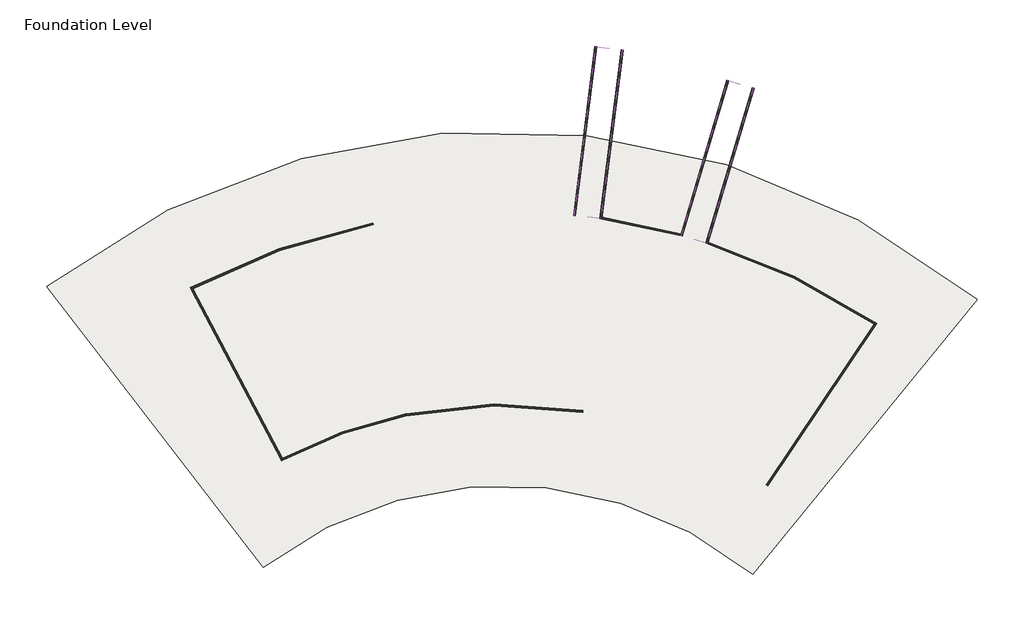
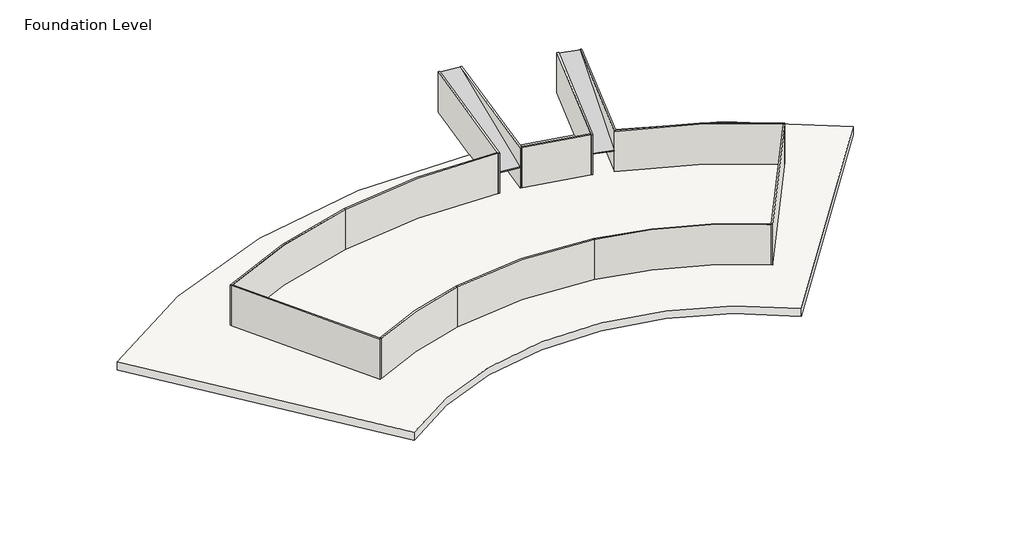
# One storey: 14 walls, 2 ramps, 1 slab.
"""IFC4 building model written with IfcOpenShell, lengths in millimetres."""

import ifcopenshell
import ifcopenshell.guid

model = None  # the IFC model being written
_history = None  # IfcOwnerHistory: only IFC2X3 demands one
_inside = {}  # id of a spatial element -> (the spatial element, [elements in it])
_under = {}  # id of a project, library or spatial element -> (it, [spatial elements below it])
_declared = {}  # id of a project -> (the project, [libraries it declares])
_typed = {}  # id of a type object -> (the type object, [elements of that type])
_made_of = {}  # id of a material, layer set ... -> (it, [elements and type objects made of it])


def new_model(schema):
    """Start an empty IFC model of exactly this schema.

    Asked for "IFC4X3", IfcOpenShell would pick the latest addendum, in which some entities
    have other attributes; the version numbers below select the first issue.
    IFC2X3 requires an IfcOwnerHistory on every rooted entity: one is made here for all.
    """
    global model, _history
    if schema == "IFC4X3":
        model = ifcopenshell.file(schema_version=(4, 3, 0, 0))
    else:
        model = ifcopenshell.file(schema=schema)
    _inside.clear()
    _under.clear()
    _declared.clear()
    _typed.clear()
    _made_of.clear()
    _history = None
    if model.schema == "IFC2X3":
        org = make("IfcOrganization", Name="unknown")
        user = make(
            "IfcPersonAndOrganization",
            ThePerson=make("IfcPerson", FamilyName="unknown"),
            TheOrganization=org,
        )
        app = make(
            "IfcApplication",
            ApplicationDeveloper=org,
            Version="unknown",
            ApplicationFullName="unknown",
            ApplicationIdentifier="unknown",
        )
        _history = make(
            "IfcOwnerHistory",
            OwningUser=user,
            OwningApplication=app,
            ChangeAction="ADDED",
            CreationDate=0,
        )
    return model


def make(cls, **values):
    """One entity of the class cls with the attributes given. An attribute that is None is left unset."""
    return model.create_entity(
        cls, **{name: value for name, value in values.items() if value is not None}
    )


def rooted(cls, **values):
    """An entity with a GlobalId (a new one), such as an element, a storey or a relation."""
    return make(cls, GlobalId=ifcopenshell.guid.new(), OwnerHistory=_history, **values)


def si_unit(unit_type, name, prefix=None):
    """IfcSIUnit, for example si_unit("LENGTHUNIT", "METRE", prefix="MILLI")."""
    return make("IfcSIUnit", UnitType=unit_type, Prefix=prefix, Name=name)


def assignment(units):
    """IfcUnitAssignment: the units of a project."""
    return None if units is None else make("IfcUnitAssignment", Units=units)


def point(xyz):
    """IfcCartesianPoint."""
    return None if xyz is None else make("IfcCartesianPoint", Coordinates=xyz)


def direction(xyz):
    """IfcDirection."""
    return None if xyz is None else make("IfcDirection", DirectionRatios=xyz)


def frame(location, z_axis=None, x_axis=None):
    """IfcAxis2Placement3D, a coordinate frame: its origin and axes. An axis left out is left unset."""
    return make(
        "IfcAxis2Placement3D",
        Location=point(location),
        Axis=direction(z_axis),
        RefDirection=direction(x_axis),
    )


def frame_2d(location, x_axis=None):
    """IfcAxis2Placement2D, a coordinate frame in the plane: its origin and x axis."""
    return make(
        "IfcAxis2Placement2D", Location=point(location), RefDirection=direction(x_axis)
    )


def origin():
    """The frame at (0, 0, 0) with its axes left unset."""
    return frame((0.0, 0.0, 0.0))


def origin_2d():
    """The frame at (0, 0) in the plane with its x axis left unset."""
    return frame_2d((0.0, 0.0))


def place(relative_to, where):
    """IfcLocalPlacement: puts the frame where relative to a parent placement (None: the world)."""
    return make(
        "IfcLocalPlacement", PlacementRelTo=relative_to, RelativePlacement=where
    )


def context(
    kind, dimensions, precision=None, world=None, true_north=None, identifier=None
):
    """IfcGeometricRepresentationContext, for example the 3D "Model" context."""
    return make(
        "IfcGeometricRepresentationContext",
        ContextIdentifier=identifier,
        ContextType=kind,
        CoordinateSpaceDimension=dimensions,
        Precision=precision,
        WorldCoordinateSystem=world,
        TrueNorth=true_north,
    )


def project(units=None, contexts=None):
    """IfcProject with its units and contexts."""
    return rooted(
        "IfcProject",
        Name="project",
        RepresentationContexts=contexts,
        UnitsInContext=assignment(units),
    )


def spatial(cls, under=None, at=None, **own):
    """A site, building, storey or space (cls), placed at a placement, below another one or the project."""
    s = rooted(cls, ObjectPlacement=at, **own)
    if under is not None:
        _under.setdefault(under.id(), (under, []))[1].append(s)
    return s


def polyline(points):
    """IfcPolyline through the points."""
    return make("IfcPolyline", Points=[point(p) for p in points])


def circle_curve(where, radius):
    """IfcCircle in the frame where."""
    return make("IfcCircle", Position=where, Radius=radius)


def trimmed(basis, trim1, trim2, sense, master):
    """IfcTrimmedCurve: the piece of a basis curve between two trims."""
    return make(
        "IfcTrimmedCurve",
        BasisCurve=basis,
        Trim1=trim1,
        Trim2=trim2,
        SenseAgreement=sense,
        MasterRepresentation=master,
    )


def segment(curve, same_sense, transition):
    """IfcCompositeCurveSegment."""
    return make(
        "IfcCompositeCurveSegment",
        Transition=transition,
        SameSense=same_sense,
        ParentCurve=curve,
    )


def composite_curve(segments, self_intersect=None):
    """IfcCompositeCurve: segments joined end to end."""
    return make("IfcCompositeCurve", Segments=segments, SelfIntersect=self_intersect)


def outline(outer, holes=None, kind="AREA"):
    """IfcArbitraryClosedProfileDef: a profile drawn as a closed curve; with holes, ...WithVoids."""
    if holes is None:
        return make("IfcArbitraryClosedProfileDef", ProfileType=kind, OuterCurve=outer)
    return make(
        "IfcArbitraryProfileDefWithVoids",
        ProfileType=kind,
        OuterCurve=outer,
        InnerCurves=holes,
    )


def extrude(swept, where, along, depth):
    """IfcExtrudedAreaSolid: the profile swept, set in the frame where, extruded along a direction by depth."""
    return make(
        "IfcExtrudedAreaSolid",
        SweptArea=swept,
        Position=where,
        ExtrudedDirection=direction(along),
        Depth=depth,
    )


def shape(context_of_items, identifier, shape_type, items):
    """IfcShapeRepresentation: the items that make up one representation, for example the "Body"."""
    return make(
        "IfcShapeRepresentation",
        ContextOfItems=context_of_items,
        RepresentationIdentifier=identifier,
        RepresentationType=shape_type,
        Items=items,
    )


def source(mapping_origin, context_of_items, identifier, shape_type, items):
    """IfcRepresentationMap: a shape defined once, which mapped items show again and again."""
    return make(
        "IfcRepresentationMap",
        MappingOrigin=mapping_origin,
        MappedRepresentation=shape(context_of_items, identifier, shape_type, items),
    )


def transform(
    local_origin,
    x_axis=None,
    y_axis=None,
    z_axis=None,
    scale=None,
    scale2=None,
    scale3=None,
    uniform=True,
):
    """IfcCartesianTransformationOperator3D, or its non-uniform kind. x_axis, y_axis, z_axis: its Axis1, 2, 3."""
    if uniform:
        return make(
            "IfcCartesianTransformationOperator3D",
            Axis1=direction(x_axis),
            Axis2=direction(y_axis),
            LocalOrigin=point(local_origin),
            Scale=scale,
            Axis3=direction(z_axis),
        )
    return make(
        "IfcCartesianTransformationOperator3DnonUniform",
        Axis1=direction(x_axis),
        Axis2=direction(y_axis),
        LocalOrigin=point(local_origin),
        Scale=scale,
        Axis3=direction(z_axis),
        Scale2=scale2,
        Scale3=scale3,
    )


def mapped(mapping_source, mapping_target):
    """IfcMappedItem: shows the shape of a source again, moved by a transform."""
    return make(
        "IfcMappedItem", MappingSource=mapping_source, MappingTarget=mapping_target
    )


def made_of(thing, what):
    """Note that an element or type object is made of a material, layer set ...; save() writes the relation."""
    if what is not None:
        _made_of.setdefault(what.id(), (what, []))[1].append(thing)
    return thing


def element(
    cls,
    number,
    at=None,
    inside=None,
    cuts=None,
    type_object=None,
    material=None,
    context=None,
    identifier="Body",
    shape_type=None,
    held_by="IfcProductDefinitionShape",
    body=None,
    shapes=None,
    **own,
):
    """One element of the class cls, such as IfcWall. Its Tag is "e" and its number.

    at: its placement. inside: the storey or other place that contains it. cuts: it is an
    opening in that element (IfcRelVoidsElement). A single representation is given by context,
    identifier, shape_type and body (its items); several are given by shapes. held_by: the class
    of the entity that holds the representations. save() writes the other relations.
    """
    e = rooted(cls, Tag="e%d" % number, ObjectPlacement=at, **own)
    if body is not None:
        shapes = [shape(context, identifier, shape_type, body)]
    if shapes is not None:
        e.Representation = make(held_by, Representations=shapes)
    if inside is not None:
        _inside.setdefault(inside.id(), (inside, []))[1].append(e)
    if cuts is not None:
        rooted(
            "IfcRelVoidsElement", RelatingBuildingElement=cuts, RelatedOpeningElement=e
        )
    if type_object is not None:
        _typed.setdefault(type_object.id(), (type_object, []))[1].append(e)
    return made_of(e, material)


def aggregate(whole, parts):
    """IfcRelAggregates: a whole, such as a stair, and the parts it consists of."""
    return rooted("IfcRelAggregates", RelatingObject=whole, RelatedObjects=parts)


def save(model, path):
    """Write the relations noted so far, then the file.

    IfcRelAggregates (storeys below a building ...), IfcRelContainedInSpatialStructure (elements
    in a storey), IfcRelDefinesByType, IfcRelAssociatesMaterial and IfcRelDeclares: one each for
    every whole, place, type object, material and project.
    """
    for whole, parts in _under.values():
        aggregate(whole, parts)
    for where, things in _inside.values():
        rooted(
            "IfcRelContainedInSpatialStructure",
            RelatedElements=things,
            RelatingStructure=where,
        )
    for kind, things in _typed.values():
        rooted("IfcRelDefinesByType", RelatedObjects=things, RelatingType=kind)
    for what, things in _made_of.values():
        rooted("IfcRelAssociatesMaterial", RelatedObjects=things, RelatingMaterial=what)
    for by, libraries in _declared.values():
        rooted("IfcRelDeclares", RelatingContext=by, RelatedDefinitions=libraries)
    model.write(path)


def plane_surface(at):
    """IfcPlane: the flat surface through the origin of the frame at, square to its z axis."""
    return make("IfcPlane", Position=at)


def cylinder_surface(at, radius):
    """IfcCylindricalSurface: all points at the distance radius from the z axis of the frame at."""
    return make("IfcCylindricalSurface", Position=at, Radius=radius)


def revolved_surface(curve, axis_point, axis_direction):
    """IfcSurfaceOfRevolution: the curve turned about the line through axis_point along axis_direction."""
    return make(
        "IfcSurfaceOfRevolution",
        SweptCurve=make("IfcArbitraryOpenProfileDef", ProfileType="CURVE", Curve=curve),
        AxisPosition=make("IfcAxis1Placement", Location=point(axis_point), Axis=direction(axis_direction)),
    )


def advanced_brep(points, edges, surfaces, faces):
    """IfcAdvancedBrep: a solid bounded by faces that lie on surfaces and meet in shared edges.

    An edge is (start, end): straight between two places in points (the first is 0);
    or (start, end, curve); or (start, end, curve, False) where it runs against its curve.
    A face is (place in surfaces, loops), or (place, loops, False) where it looks against
    its surface's normal. A loop lists edges by number (the first is 1), with a minus sign
    where the edge is run from its end to its start. The first loop is the outer one.
    """
    corners = [point(p) for p in points]
    vertices = [make("IfcVertexPoint", VertexGeometry=c) for c in corners]
    made = []
    for start, end, *more in edges:
        made.append(
            make(
                "IfcEdgeCurve",
                EdgeStart=vertices[start],
                EdgeEnd=vertices[end],
                EdgeGeometry=more[0] if more else make("IfcPolyline", Points=[corners[start], corners[end]]),
                SameSense=more[1] if len(more) > 1 else True,
            )
        )
    hull = []
    for where, loops, *sense in faces:
        bounds = []
        for j, loop in enumerate(loops):
            ring = [make("IfcOrientedEdge", EdgeElement=made[abs(k) - 1], Orientation=k > 0) for k in loop]
            bounds.append(
                make(
                    "IfcFaceOuterBound" if j == 0 else "IfcFaceBound",
                    Bound=make("IfcEdgeLoop", EdgeList=ring),
                    Orientation=True,
                )
            )
        hull.append(make("IfcAdvancedFace", Bounds=bounds, FaceSurface=surfaces[where], SameSense=sense[0] if sense else True))
    return make("IfcAdvancedBrep", Outer=make("IfcClosedShell", CfsFaces=hull))


def ramp_1_e6d8d0b2(model_context):
    return source(origin(), model_context, "Body", "SweptSolid", [
        extrude(outline(polyline([(-4700.0, -30704.1914312), (0.0, 0.0), (202.3295842, 0.0), (-4497.6704158, -30704.1914312), (-4700.0, -30704.1914312)])), frame((38391.793903, 120222.1050221, 5300.0), z_axis=(-0.9584455062260432, 0.28527567648697966, 0.0), x_axis=(0.0, 0.0, -1.0)), (0.0, 0.0, 1.0), 5000.0),
    ])


def ramp_1_3ccef93f(model_context):
    return source(origin(), model_context, "Body", "SweptSolid", [
        extrude(outline(polyline([(-4700.0, -32182.9414905), (0.0, 0.0), (202.121519, 0.0), (-4497.878481, -32182.9414905), (-4700.0, -32182.9414905)])), frame((18351.118119, 124883.6460283, 5300.0), z_axis=(-0.9920606394423034, 0.12576043761584285, 0.0), x_axis=(0.0, 0.0, -1.0)), (0.0, 0.0, 1.0), 5000.0),
    ])


model = new_model("IFC4")

# Units and contexts
model_context = context("Model", 3, world=origin())
ifc_project = project(units=[si_unit("LENGTHUNIT", "METRE", prefix="MILLI")], contexts=[model_context])

# Site, building, storey
site = spatial("IfcSite", under=ifc_project)
building = spatial("IfcBuilding", under=site)
storey = spatial("IfcBuildingStorey", under=building, Name="Foundation Level", Elevation=-100.0)

# Ramps
placement = place(None, origin())
ramp_1_shape = ramp_1_e6d8d0b2(model_context)
element("IfcRamp", 1, ObjectType="Ramp 1", at=placement, inside=storey, context=model_context, shape_type="MappedRepresentation", body=[
    mapped(ramp_1_shape, transform((0.0, 0.0, 0.0), x_axis=(1.0, 0.0, 0.0), y_axis=(0.0, 1.0, 0.0), z_axis=(0.0, 0.0, 1.0))),
])
ramp_1_2_shape = ramp_1_3ccef93f(model_context)
element("IfcRamp", 2, ObjectType="Ramp 1", at=placement, inside=storey, context=model_context, shape_type="MappedRepresentation", body=[
    mapped(ramp_1_2_shape, transform((0.0, 0.0, 0.0), x_axis=(1.0, 0.0, 0.0), y_axis=(0.0, 1.0, 0.0), z_axis=(0.0, 0.0, 1.0))),
])

# Slab
element("IfcSlab", 3, ObjectType="2000mm Foundation Slab", at=placement, inside=storey, context=model_context, shape_type="SweptSolid", body=[
    extrude(outline(composite_curve([segment(polyline([(89534.4922579, 109576.6624408), (47102.2655432, 57646.0414469)]), True, "CONTINUOUS"), segment(trimmed(circle_curve(origin_2d(), 74442.5249021), [point((47102.2655432, 57646.0414469))], [point((-45430.5356945, 58972.5015606))], True, "CARTESIAN"), True, "CONTINUOUS"), segment(polyline([(-45430.5356945, 58972.5015606), (-86356.7845729, 112098.0753395)]), True, "CONTINUOUS"), segment(trimmed(circle_curve(frame_2d((-0.0516599, -3.1117517)), 141506.754138), [point((-86356.7845729, 112098.0753395))], [point((89534.4922579, 109576.6624408))], False, "CARTESIAN"), True, "CONTINUOUS")], self_intersect=False)), frame((0.0, 0.0, -2100.0), z_axis=(0.0, 0.0, 1.0), x_axis=(1.0, 0.0, 0.0)), (0.0, 0.0, 1.0), 2000.0),
])

# Walls
element("IfcWall", 4, ObjectType="Retaining - 350mm Concrete", at=placement, inside=storey, context=model_context, shape_type="AdvancedBrep", body=[
    advanced_brep(
    [(-24695.8381961, 124116.9532167, 10150.0), (-59193.8326032, 111852.5488388, 10150.0), (-59030.4865839, 111543.003607, 10150.0), (-58720.9027462, 111706.2915448, 10150.0), (-24627.5367867, 123773.682307, 10150.0), (-24695.8381961, 124116.9532167, -100.0), (-24627.5367867, 123773.682307, -100.0), (-58720.9027462, 111706.2915448, -100.0), (-59030.4865839, 111543.003607, -100.0), (-59193.8326032, 111852.5488388, -100.0)],
    [
        (0, 1, circle_curve(frame((0.0, 0.0, 10150.0), z_axis=(0.0, 0.0, 1.0), x_axis=(-0.20635882667529443, 0.9784763843104216, 0.0)), 126550.0)),
        (1, 2),
        (2, 3, circle_curve(frame((0.0, 0.0, 10150.0), z_axis=(0.0, 0.0, -1.0), x_axis=(-0.20635882667529443, 0.9784763843104216, 0.0)), 126200.0)),
        (3, 4, circle_curve(frame((0.0, 0.0, 10150.0), z_axis=(0.0, 0.0, -1.0), x_axis=(-0.20635882667529443, 0.9784763843104216, 0.0)), 126199.9999605)),
        (4, 0),
        (5, 6),
        (6, 7, circle_curve(frame((0.0, 0.0, -100.0), z_axis=(0.0, 0.0, 1.0), x_axis=(-0.20635882667529443, 0.9784763843104216, 0.0)), 126200.0)),
        (7, 8, circle_curve(frame((0.0, 0.0, -100.0), z_axis=(0.0, 0.0, 1.0), x_axis=(-0.20635882667529443, 0.9784763843104216, 0.0)), 126199.9999605)),
        (8, 9),
        (9, 5, circle_curve(frame((0.0, 0.0, -100.0), z_axis=(0.0, 0.0, -1.0), x_axis=(-0.20635882667529443, 0.9784763843104216, 0.0)), 126550.0)),
        (0, 5),
        (9, 1),
        (2, 8),
        (6, 4),
    ],
    [
        plane_surface(frame((-26114.7095158, 123826.1864345, 10150.0), z_axis=(0.0, 0.0, 1.0), x_axis=(-0.9784763843104216, -0.2063588266752944, 0.0))),
        plane_surface(frame((-26114.7095158, 123826.1864345, -100.0), z_axis=(0.0, 0.0, -1.0), x_axis=(0.9784763843104216, 0.2063588266752944, 0.0))),
        cylinder_surface(frame((0.0, 0.0, -100.0), z_axis=(0.0, 0.0, 1.0000000000000002), x_axis=(-0.20635882667529443, 0.9784763843104216, 0.0)), 126550.0),
        revolved_surface(polyline([(-26042.483926422155, 123483.7196999752, -100.0), (-26042.483926422155, 123483.7196999752, 10150.000000000004)]), (0.0, 0.0, -100.0), (0.0, 0.0, -1.0000000000000002)),
        plane_surface(frame((-24627.5367867, 123773.682307, 10150.0), z_axis=(0.9807740277892864, 0.19514688420259294, 0.0), x_axis=(0.0, 0.0, -1.0))),
        plane_surface(frame((-59193.8326032, 111852.5488388, -100.0), z_axis=(-0.8844143251580528, -0.4667025835103401, 0.0), x_axis=(0.4667025835103401, -0.8844143251580528, 0.0))),
    ],
    [
        (0, [[1, 2, 3, 4, 5]]),
        (1, [[6, 7, 8, 9, 10]]),
        (2, [[-1, 11, -10, 12]]),
        (3, [[-4, -3, 13, -8, -7, 14]]),
        (4, [[-5, -14, -6, -11]]),
        (5, [[-2, -12, -9, -13]]),
    ],
),
])
element("IfcWall", 5, ObjectType="Retaining - 350mm Concrete", at=placement, inside=storey, context=model_context, shape_type="AdvancedBrep", body=[
    advanced_brep(
    [(-41616.2292553, 79292.4458102, -100.0), (-41779.5755654, 79601.991593, -100.0), (-58720.9092116, 111706.2881908, -100.0), (-58720.9092116, 111706.2881908, 10150.0), (-41779.5755654, 79601.991593, 10150.0), (-41616.2292553, 79292.4458102, 10150.0), (-41925.8198711, 79129.186323, -100.0), (-41925.8198711, 79129.186323, 10150.0), (-59030.4865839, 111543.003607, 10150.0), (-59030.4865839, 111543.003607, -100.0)],
    [
        (0, 1),
        (1, 2),
        (2, 3),
        (3, 4),
        (4, 5),
        (5, 0),
        (6, 7),
        (7, 8),
        (8, 9),
        (9, 6),
        (0, 6, circle_curve(frame((0.0, 0.0, -100.0), z_axis=(0.0, 0.0, 1.0), x_axis=(1.0, 0.0, 0.0)), 89550.0)),
        (9, 2, circle_curve(frame((0.0, 0.0, -100.0), z_axis=(0.0, 0.0, -1.0), x_axis=(-0.20635882667529443, 0.9784763843104216, 0.0)), 126200.0)),
        (3, 8, circle_curve(frame((0.0, 0.0, 10150.0), z_axis=(0.0, 0.0, 1.0), x_axis=(-0.20635882667529443, 0.9784763843104216, 0.0)), 126200.0)),
        (7, 5, circle_curve(frame((0.0, 0.0, 10150.0), z_axis=(0.0, 0.0, -1.0), x_axis=(1.0, 0.0, 0.0)), 89550.0)),
    ],
    [
        plane_surface(frame((-58884.2875894, 112015.8947431, -100.0), z_axis=(0.8844143251580528, 0.4667025835103401, 0.0), x_axis=(-0.4667025835103401, 0.8844143251580528, 0.0))),
        plane_surface(frame((-59193.8326032, 111852.5488388, -100.0), z_axis=(-0.8844143251580528, -0.4667025835103401, 0.0), x_axis=(0.4667025835103401, -0.8844143251580528, 0.0))),
        plane_surface(frame((-41698.004815, 79447.4127612, -100.0), z_axis=(0.0, 0.0, -1.0), x_axis=(-0.8844143251580571, -0.46670258351033217, 0.0))),
        plane_surface(frame((-58802.654972, 111861.1986716, 10150.0), z_axis=(0.0, 0.0, 1.0000000000000002), x_axis=(-0.8844143251580625, -0.46670258351032196, 0.0))),
        cylinder_surface(frame((0.0, 0.0, -100.0), z_axis=(0.0, 0.0, -1.0000000000000002), x_axis=(-0.20635882667529443, 0.9784763843104216, 0.0)), 126200.0),
        revolved_surface(polyline([(89550.0, 0.0, -100.0), (89550.0, 0.0, 10150.0)]), (0.0, 0.0, -100.0), (0.0, 0.0, -1.0)),
    ],
    [
        (0, [[1, 2, 3, 4, 5, 6]]),
        (1, [[7, 8, 9, 10]]),
        (2, [[-2, -1, 11, -10, 12]]),
        (3, [[-5, -4, 13, -8, 14]]),
        (4, [[-3, -12, -9, -13]]),
        (5, [[-6, -14, -7, -11]]),
    ],
),
])
element("IfcWall", 6, ObjectType="Retaining - 350mm Concrete", at=placement, inside=storey, context=model_context, shape_type="SweptSolid", body=[
    extrude(outline(composite_curve([segment(polyline([(-18557.3915102, 87963.8176771), (-18485.1436011, 87621.3556506)]), True, "CONTINUOUS"), segment(trimmed(circle_curve(origin_2d(), 89550.0), [point((-18485.1436011, 87621.3556506))], [point((-41616.2292553, 79292.4458102))], True, "CARTESIAN"), True, "CONTINUOUS"), segment(polyline([(-41616.2292553, 79292.4458102), (-41779.5755654, 79601.991593)]), True, "CONTINUOUS"), segment(trimmed(circle_curve(origin_2d(), 89900.0), [point((-41779.5755654, 79601.991593))], [point((-18557.3915102, 87963.8176771))], False, "CARTESIAN"), True, "CONTINUOUS")], self_intersect=False)), frame((0.0, 0.0, -100.0), z_axis=(0.0, 0.0, 1.0), x_axis=(1.0, 0.0, 0.0)), (0.0, 0.0, 1.0), 10250.0),
])
element("IfcWall", 7, ObjectType="Retaining - 350mm Concrete", at=placement, inside=storey, context=model_context, shape_type="SweptSolid", body=[
    extrude(outline(composite_curve([segment(polyline([(14972.724009, 88644.3880669), (14914.4319801, 88299.2764337)]), True, "CONTINUOUS"), segment(trimmed(circle_curve(origin_2d(), 89550.0), [point((14914.4319801, 88299.2764337))], [point((-18446.0903575, 87629.585475))], True, "CARTESIAN"), True, "CONTINUOUS"), segment(polyline([(-18446.0903575, 87629.585475), (-18518.1856297, 87972.0796673)]), True, "CONTINUOUS"), segment(trimmed(circle_curve(origin_2d(), 89900.0), [point((-18518.1856297, 87972.0796673))], [point((14972.724009, 88644.3880669))], False, "CARTESIAN"), True, "CONTINUOUS")], self_intersect=False)), frame((0.0, 0.0, -100.0), z_axis=(0.0, 0.0, 1.0), x_axis=(1.0, 0.0, 0.0)), (0.0, 0.0, 1.0), 10250.0),
])
element("IfcWall", 8, ObjectType="Retaining - 350mm Concrete", at=placement, inside=storey, context=model_context, shape_type="SweptSolid", body=[
    extrude(outline(composite_curve([segment(polyline([(49779.3599905, 74860.0381975), (49584.131796, 74569.5405245)]), True, "CONTINUOUS"), segment(trimmed(circle_curve(origin_2d(), 89550.0), [point((49584.131796, 74569.5405245))], [point((14953.8498127, 88292.6094063))], True, "CARTESIAN"), True, "CONTINUOUS"), segment(polyline([(14953.8498127, 88292.6094063), (15012.2959035, 88637.6949819)]), True, "CONTINUOUS"), segment(trimmed(circle_curve(origin_2d(), 89900.0), [point((15012.2959035, 88637.6949819))], [point((49779.3599905, 74860.0381975))], False, "CARTESIAN"), True, "CONTINUOUS")], self_intersect=False)), frame((0.0, 0.0, -100.0), z_axis=(0.0, 0.0, 1.0), x_axis=(1.0, 0.0, 0.0)), (0.0, 0.0, 1.0), 10250.0),
])
element("IfcWall", 9, ObjectType="Retaining - 350mm Concrete", at=placement, inside=storey, context=model_context, shape_type="AdvancedBrep", body=[
    advanced_brep(
    [(49875.2037, 74375.1743251, -100.0), (70318.1461496, 104794.0757967, -100.0), (70318.1461496, 104794.0757967, 10150.0), (49875.2037, 74375.1743251, 10150.0), (49584.131796, 74569.5405245, -100.0), (49584.131796, 74569.5405245, 10150.0), (49779.3599905, 74860.0381975, 10150.0), (70027.2420249, 104988.69165, 10150.0), (70027.2420249, 104988.69165, -100.0), (49779.3599905, 74860.0381975, -100.0)],
    [
        (0, 1),
        (1, 2),
        (2, 3),
        (3, 0),
        (4, 5),
        (5, 6),
        (6, 7),
        (7, 8),
        (8, 9),
        (9, 4),
        (0, 4, circle_curve(frame((0.0, 0.0, -100.0), z_axis=(0.0, 0.0, 1.0), x_axis=(1.0, 0.0, 0.0)), 89550.0)),
        (8, 1, circle_curve(frame((0.0, 0.0, -100.0), z_axis=(0.0, 0.0, -1.0), x_axis=(1.0, 0.0, 0.0)), 126200.0)),
        (2, 7, circle_curve(frame((0.0, 0.0, 10150.0), z_axis=(0.0, 0.0, 1.0), x_axis=(1.0, 0.0, 0.0)), 126200.0)),
        (5, 3, circle_curve(frame((0.0, 0.0, 10150.0), z_axis=(0.0, 0.0, -1.0), x_axis=(1.0, 0.0, 0.0)), 89550.0)),
    ],
    [
        plane_surface(frame((53500.2736927, 79769.2435598, -100.0), z_axis=(0.8299833716350299, -0.557788134338969, 0.0), x_axis=(0.557788134338969, 0.8299833716350299, 0.0))),
        plane_surface(frame((53209.7795126, 79964.4694068, -100.0), z_axis=(-0.8299833716350299, 0.557788134338969, 0.0), x_axis=(-0.557788134338969, -0.8299833716350299, 0.0))),
        plane_surface(frame((49972.6235678, 74520.1341501, -100.0), z_axis=(0.0, 0.0, -1.0), x_axis=(-0.8299833716350266, 0.5577881343389741, 0.0))),
        plane_surface(frame((70415.6219955, 104939.1189165, 10150.0), z_axis=(0.0, 0.0, 1.0), x_axis=(-0.829983371635038, 0.557788134338957, 0.0))),
        cylinder_surface(frame((0.0, 0.0, -100.0), z_axis=(0.0, 0.0, -1.0), x_axis=(1.0, 0.0, 0.0)), 126200.0),
        revolved_surface(polyline([(89550.0, 0.0, -100.0), (89550.0, 0.0, 10150.0)]), (0.0, 0.0, -100.0), (0.0, 0.0, -1.0)),
    ],
    [
        (0, [[1, 2, 3, 4]]),
        (1, [[5, 6, 7, 8, 9, 10]]),
        (2, [[-1, 11, -10, -9, 12]]),
        (3, [[-3, 13, -7, -6, 14]]),
        (4, [[-2, -12, -8, -13]]),
        (5, [[-4, -14, -5, -11]]),
    ],
),
])
element("IfcWall", 10, ObjectType="Retaining - 350mm Concrete", at=placement, inside=storey, context=model_context, shape_type="AdvancedBrep", body=[
    advanced_brep(
    [(70513.3720462, 105084.5700504, 10150.0), (38657.4189135, 120501.0641191, 10150.0), (38323.9293281, 120607.5409784, 10150.0), (38224.0659394, 120272.0282654, 10150.0), (70027.2363144, 104988.6954158, 10150.0), (70318.1461496, 104794.0757967, 10150.0), (70513.3720462, 105084.5700504, -100.0), (70318.1461496, 104794.0757967, -100.0), (70027.2363144, 104988.6954158, -100.0), (38224.0659394, 120272.0282654, -100.0), (38323.9293281, 120607.5409784, -100.0), (38657.4189135, 120501.0641191, -100.0)],
    [
        (0, 1, circle_curve(frame((0.0, 0.0, 10150.0), z_axis=(0.0, 0.0, 1.0), x_axis=(1.0, 0.0, 0.0)), 126550.0)),
        (1, 2, circle_curve(frame((0.0, 0.0, 10150.0), z_axis=(0.0, 0.0, 1.0), x_axis=(1.0, 0.0, 0.0)), 126549.999964)),
        (2, 3),
        (3, 4, circle_curve(frame((0.0, 0.0, 10150.0), z_axis=(0.0, 0.0, -1.0), x_axis=(1.0, 0.0, 0.0)), 126200.0)),
        (4, 5, circle_curve(frame((0.0, 0.0, 10150.0), z_axis=(0.0, 0.0, -1.0), x_axis=(1.0, 0.0, 0.0)), 126199.9999641)),
        (5, 0),
        (6, 7),
        (7, 8, circle_curve(frame((0.0, 0.0, -100.0), z_axis=(0.0, 0.0, 1.0), x_axis=(1.0, 0.0, 0.0)), 126200.0)),
        (8, 9, circle_curve(frame((0.0, 0.0, -100.0), z_axis=(0.0, 0.0, 1.0), x_axis=(1.0, 0.0, 0.0)), 126199.9999641)),
        (9, 10),
        (10, 11, circle_curve(frame((0.0, 0.0, -100.0), z_axis=(0.0, 0.0, -1.0), x_axis=(1.0, 0.0, 0.0)), 126550.0)),
        (11, 6, circle_curve(frame((0.0, 0.0, -100.0), z_axis=(0.0, 0.0, -1.0), x_axis=(1.0, 0.0, 0.0)), 126549.999964)),
        (0, 6),
        (10, 2),
        (3, 9),
        (7, 5),
    ],
    [
        plane_surface(frame((126550.0, 0.0, 10150.0), z_axis=(0.0, 0.0, 1.0), x_axis=(0.0, 1.0, 0.0))),
        plane_surface(frame((126550.0, 0.0, -100.0), z_axis=(0.0, 0.0, -1.0), x_axis=(0.0, -1.0, 0.0))),
        cylinder_surface(frame((0.0, 0.0, -100.0), z_axis=(0.0, 0.0, 1.0), x_axis=(1.0, 0.0, 0.0)), 126550.0),
        revolved_surface(polyline([(126200.0, 0.0, -100.0), (126200.0, 0.0, 10150.0)]), (0.0, 0.0, -100.0), (0.0, 0.0, -1.0)),
        plane_surface(frame((41572.3875987, 131521.4410696, -100.0), z_axis=(-0.9584455062260441, 0.2852756764869767, 0.0), x_axis=(-0.2852756764869767, -0.9584455062260441, 0.0))),
        plane_surface(frame((53500.2736927, 79769.2435598, -100.0), z_axis=(0.8299833716350299, -0.557788134338969, 0.0), x_axis=(0.557788134338969, 0.8299833716350299, 0.0))),
    ],
    [
        (0, [[1, 2, 3, 4, 5, 6]]),
        (1, [[7, 8, 9, 10, 11, 12]]),
        (2, [[-2, -1, 13, -12, -11, 14]]),
        (3, [[-5, -4, 15, -9, -8, 16]]),
        (4, [[-3, -14, -10, -15]]),
        (5, [[-6, -16, -7, -13]]),
    ],
),
])
element("IfcWall", 11, ObjectType="Retaining - 350mm Concrete", at=placement, inside=storey, context=model_context, shape_type="SweptSolid", body=[
    extrude(outline(composite_curve([segment(polyline([(38323.9293281, 120607.5409784), (46983.2249209, 149700.322565), (47318.6808481, 149600.4760782), (38657.4123973, 120501.0662473)]), True, "CONTINUOUS"), segment(trimmed(circle_curve(origin_2d(), 126550.0), [point((38657.4123973, 120501.0662473))], [point((38323.9293281, 120607.5409784))], True, "CARTESIAN"), True, "CONTINUOUS")], self_intersect=False)), frame((0.0, 0.0, -100.0), z_axis=(0.0, 0.0, 1.0), x_axis=(1.0, 0.0, 0.0)), (0.0, 0.0, 1.0), 10250.0),
])
element("IfcWall", 12, ObjectType="Retaining - 350mm Concrete", at=placement, inside=storey, context=model_context, shape_type="AdvancedBrep", body=[
    advanced_brep(
    [(33767.2943355, 121598.5601611, -100.0), (42526.453317, 151026.8544607, -100.0), (42526.453317, 151026.8544607, 10150.0), (33767.2943355, 121598.5601611, 10150.0), (33429.8600767, 121691.7600138, -100.0), (33429.8600767, 121691.7600138, 10150.0), (33529.7289391, 122027.2911167, 10150.0), (42190.9973898, 151126.7009474, 10150.0), (42190.9973898, 151126.7009474, -100.0), (33529.7289391, 122027.2911167, -100.0)],
    [
        (0, 1),
        (1, 2),
        (2, 3),
        (3, 0),
        (4, 5),
        (5, 6),
        (6, 7),
        (7, 8),
        (8, 9),
        (9, 4),
        (0, 4, circle_curve(frame((0.0, 0.0, -100.0), z_axis=(0.0, 0.0, 1.0), x_axis=(1.0, 0.0, 0.0)), 126200.0)),
        (8, 1),
        (7, 2),
        (5, 3, circle_curve(frame((0.0, 0.0, 10150.0), z_axis=(0.0, 0.0, -1.0), x_axis=(1.0, 0.0, 0.0)), 126200.0)),
    ],
    [
        plane_surface(frame((37652.8840881, 134653.0416484, -100.0), z_axis=(0.9584455062260449, -0.28527567648697416, 0.0), x_axis=(0.28527567648697416, 0.9584455062260449, 0.0))),
        plane_surface(frame((37317.4281609, 134752.8881352, -100.0), z_axis=(-0.9584455062260449, 0.28527567648697416, 0.0), x_axis=(-0.28527567648697416, -0.9584455062260449, 0.0))),
        plane_surface(frame((33816.2728324, 121763.1140441, -100.0), z_axis=(0.0, 0.0, -1.0000000000000002), x_axis=(-0.9584455062260494, 0.2852756764869589, 0.0))),
        plane_surface(frame((42526.453317, 151026.8544607, -100.0), z_axis=(0.2852756764869589, 0.9584455062260494, 0.0), x_axis=(-0.9584455062260494, 0.2852756764869589, 0.0))),
        plane_surface(frame((42526.453317, 151026.8544607, 10150.0), z_axis=(0.0, 0.0, 1.0000000000000002), x_axis=(-0.9584455062260494, 0.2852756764869589, 0.0))),
        revolved_surface(polyline([(126200.0, 0.0, -100.0), (126200.0, 0.0, 10150.0)]), (0.0, 0.0, -100.0), (0.0, 0.0, -1.0)),
    ],
    [
        (0, [[1, 2, 3, 4]]),
        (1, [[5, 6, 7, 8, 9, 10]]),
        (2, [[-1, 11, -10, -9, 12]]),
        (3, [[-2, -12, -8, 13]]),
        (4, [[-3, -13, -7, -6, 14]]),
        (5, [[-4, -14, -5, -11]]),
    ],
),
])
element("IfcWall", 13, ObjectType="Retaining - 350mm Concrete", at=placement, inside=storey, context=model_context, shape_type="AdvancedBrep", body=[
    advanced_brep(
    [(70513.3720462, 105084.5700504, 10150.0), (38657.4189135, 120501.0641191, 10150.0), (38323.9293281, 120607.5409784, 10150.0), (38224.0659394, 120272.0282654, 10150.0), (70027.2363144, 104988.6954158, 10150.0), (70318.1461496, 104794.0757967, 10150.0), (70513.3720462, 105084.5700504, -100.0), (70318.1461496, 104794.0757967, -100.0), (70027.2363144, 104988.6954158, -100.0), (38224.0659394, 120272.0282654, -100.0), (38323.9293281, 120607.5409784, -100.0), (38657.4189135, 120501.0641191, -100.0)],
    [
        (0, 1, circle_curve(frame((0.0, 0.0, 10150.0), z_axis=(0.0, 0.0, 1.0), x_axis=(1.0, 0.0, 0.0)), 126550.0)),
        (1, 2, circle_curve(frame((0.0, 0.0, 10150.0), z_axis=(0.0, 0.0, 1.0), x_axis=(1.0, 0.0, 0.0)), 126549.999964)),
        (2, 3),
        (3, 4, circle_curve(frame((0.0, 0.0, 10150.0), z_axis=(0.0, 0.0, -1.0), x_axis=(1.0, 0.0, 0.0)), 126200.0)),
        (4, 5, circle_curve(frame((0.0, 0.0, 10150.0), z_axis=(0.0, 0.0, -1.0), x_axis=(1.0, 0.0, 0.0)), 126199.9999641)),
        (5, 0),
        (6, 7),
        (7, 8, circle_curve(frame((0.0, 0.0, -100.0), z_axis=(0.0, 0.0, 1.0), x_axis=(1.0, 0.0, 0.0)), 126200.0)),
        (8, 9, circle_curve(frame((0.0, 0.0, -100.0), z_axis=(0.0, 0.0, 1.0), x_axis=(1.0, 0.0, 0.0)), 126199.9999641)),
        (9, 10),
        (10, 11, circle_curve(frame((0.0, 0.0, -100.0), z_axis=(0.0, 0.0, -1.0), x_axis=(1.0, 0.0, 0.0)), 126550.0)),
        (11, 6, circle_curve(frame((0.0, 0.0, -100.0), z_axis=(0.0, 0.0, -1.0), x_axis=(1.0, 0.0, 0.0)), 126549.999964)),
        (0, 6),
        (10, 2),
        (3, 9),
        (7, 5),
    ],
    [
        plane_surface(frame((126550.0, 0.0, 10150.0), z_axis=(0.0, 0.0, 1.0), x_axis=(0.0, 1.0, 0.0))),
        plane_surface(frame((126550.0, 0.0, -100.0), z_axis=(0.0, 0.0, -1.0), x_axis=(0.0, -1.0, 0.0))),
        cylinder_surface(frame((0.0, 0.0, -100.0), z_axis=(0.0, 0.0, 1.0), x_axis=(1.0, 0.0, 0.0)), 126550.0),
        revolved_surface(polyline([(126200.0, 0.0, -100.0), (126200.0, 0.0, 10150.0)]), (0.0, 0.0, -100.0), (0.0, 0.0, -1.0)),
        plane_surface(frame((41572.3875987, 131521.4410696, -100.0), z_axis=(-0.9584455062260441, 0.2852756764869767, 0.0), x_axis=(-0.2852756764869767, -0.9584455062260441, 0.0))),
        plane_surface(frame((53500.2736927, 79769.2435598, -100.0), z_axis=(0.8299833716350299, -0.557788134338969, 0.0), x_axis=(0.557788134338969, 0.8299833716350299, 0.0))),
    ],
    [
        (0, [[1, 2, 3, 4, 5, 6]]),
        (1, [[7, 8, 9, 10, 11, 12]]),
        (2, [[-2, -1, 13, -12, -11, 14]]),
        (3, [[-5, -4, 15, -9, -8, 16]]),
        (4, [[-3, -14, -10, -15]]),
        (5, [[-6, -16, -7, -13]]),
    ],
),
])
element("IfcWall", 14, ObjectType="Retaining - 350mm Concrete", at=placement, inside=storey, context=model_context, shape_type="SweptSolid", body=[
    extrude(outline(composite_curve([segment(polyline([(33529.7289391, 122027.2911167), (33429.8600767, 121691.7600138)]), True, "CONTINUOUS"), segment(trimmed(circle_curve(origin_2d(), 126200.0), [point((33429.8600767, 121691.7600138))], [point((18521.1636863, 124833.515114))], True, "CARTESIAN"), True, "CONTINUOUS"), segment(polyline([(18521.1636863, 124833.515114), (18565.1897035, 125180.8141501)]), True, "CONTINUOUS"), segment(trimmed(circle_curve(origin_2d(), 126550.0), [point((18565.1897035, 125180.8141501))], [point((33529.7289391, 122027.2911167))], False, "CARTESIAN"), True, "CONTINUOUS")], self_intersect=False)), frame((0.0, 0.0, -100.0), z_axis=(0.0, 0.0, 1.0), x_axis=(1.0, 0.0, 0.0)), (0.0, 0.0, 1.0), 10250.0),
])
element("IfcWall", 15, ObjectType="Retaining - 350mm Concrete", at=placement, inside=storey, context=model_context, shape_type="AdvancedBrep", body=[
    advanced_brep(
    [(13561.7326134, 125469.1970506, -100.0), (17611.7663393, 157417.869654, -100.0), (17611.7663393, 157417.869654, 10150.0), (13561.7326134, 125469.1970506, 10150.0), (13213.6392653, 125506.3334552, -100.0), (13213.6392653, 125506.3334552, 10150.0), (13257.6652825, 125853.6324913, 10150.0), (17264.5451155, 157461.8858072, 10150.0), (17264.5451155, 157461.8858072, -100.0), (13257.6652825, 125853.6324913, -100.0)],
    [
        (0, 1),
        (1, 2),
        (2, 3),
        (3, 0),
        (4, 5),
        (5, 6),
        (6, 7),
        (7, 8),
        (8, 9),
        (9, 4),
        (0, 4, circle_curve(frame((0.0, 0.0, -100.0), z_axis=(0.0, 0.0, 1.0), x_axis=(0.1047622701105178, 0.9944972934911844, 0.0)), 126200.0)),
        (8, 1),
        (7, 2),
        (5, 3, circle_curve(frame((0.0, 0.0, 10150.0), z_axis=(0.0, 0.0, -1.0), x_axis=(0.1047622701105178, 0.9944972934911844, 0.0)), 126200.0)),
    ],
    [
        plane_surface(frame((15037.8009636, 137113.1555097, -100.0), z_axis=(0.9920606394423034, -0.12576043761584296, 0.0), x_axis=(0.12576043761584296, 0.9920606394423034, 0.0))),
        plane_surface(frame((14690.5797398, 137157.1716629, -100.0), z_axis=(-0.9920606394423034, 0.12576043761584296, 0.0), x_axis=(-0.12576043761584296, -0.9920606394423034, 0.0))),
        plane_surface(frame((13583.3242096, 125639.5222588, -100.0), z_axis=(0.0, 0.0, -1.0), x_axis=(-0.9920606394423015, 0.12576043761585723, 0.0))),
        plane_surface(frame((17611.7663393, 157417.869654, -100.0), z_axis=(0.12576043761585723, 0.9920606394423015, 0.0), x_axis=(-0.9920606394423015, 0.12576043761585723, 0.0))),
        plane_surface(frame((17611.7663393, 157417.869654, 10150.0), z_axis=(0.0, 0.0, 1.0), x_axis=(-0.9920606394423015, 0.12576043761585723, 0.0))),
        revolved_surface(polyline([(13220.998487947345, 125505.55843858747, -100.0), (13220.998487947345, 125505.55843858747, 10150.0)]), (0.0, 0.0, -100.0), (0.0, 0.0, -1.0)),
    ],
    [
        (0, [[1, 2, 3, 4]]),
        (1, [[5, 6, 7, 8, 9, 10]]),
        (2, [[-1, 11, -10, -9, 12]]),
        (3, [[-2, -12, -8, 13]]),
        (4, [[-3, -13, -7, -6, 14]]),
        (5, [[-4, -14, -5, -11]]),
    ],
),
])
element("IfcWall", 16, ObjectType="Retaining - 350mm Concrete", at=placement, inside=storey, context=model_context, shape_type="AdvancedBrep", body=[
    advanced_brep(
    [(22224.8483127, 156833.0836191, -100.0), (18174.8145868, 124884.4110157, -100.0), (18174.8145868, 124884.4110157, 10150.0), (22224.8483127, 156833.0836191, 10150.0), (22572.0695365, 156789.0674659, -100.0), (22572.0695365, 156789.0674659, 10150.0), (18565.1897035, 125180.8141501, 10150.0), (18521.1636863, 124833.515114, 10150.0), (18521.1636863, 124833.515114, -100.0), (18565.1897035, 125180.8141501, -100.0)],
    [
        (0, 1),
        (1, 2),
        (2, 3),
        (3, 0),
        (4, 5),
        (5, 6),
        (6, 7),
        (7, 8),
        (8, 9),
        (9, 4),
        (0, 4),
        (8, 1, circle_curve(frame((0.0, 0.0, -100.0), z_axis=(0.0, 0.0, 1.0), x_axis=(1.0, 0.0, 0.0)), 126200.0)),
        (2, 7, circle_curve(frame((0.0, 0.0, 10150.0), z_axis=(0.0, 0.0, -1.0), x_axis=(1.0, 0.0, 0.0)), 126200.0)),
        (5, 3),
    ],
    [
        plane_surface(frame((19887.7312775, 138396.7465296, -100.0), z_axis=(-0.9920606394423029, 0.12576043761584632, 0.0), x_axis=(-0.12576043761584632, -0.9920606394423029, 0.0))),
        plane_surface(frame((20234.9525013, 138352.7303764, -100.0), z_axis=(0.9920606394423029, -0.12576043761584632, 0.0), x_axis=(0.12576043761584632, 0.9920606394423029, 0.0))),
        plane_surface(frame((22224.8483127, 156833.0836191, -100.0), z_axis=(0.0, 0.0, -1.0), x_axis=(0.9920606394423015, -0.12576043761585723, 0.0))),
        plane_surface(frame((18196.406183, 125054.7362239, 10150.0), z_axis=(0.0, 0.0, 1.0), x_axis=(0.9920606394423015, -0.12576043761585723, 0.0))),
        plane_surface(frame((22224.8483127, 156833.0836191, 10150.0), z_axis=(0.12576043761585723, 0.9920606394423015, 0.0), x_axis=(0.9920606394423015, -0.12576043761585723, 0.0))),
        revolved_surface(polyline([(126200.0, 0.0, -100.0), (126200.0, 0.0, 10150.0)]), (0.0, 0.0, -100.0), (0.0, 0.0, -1.0)),
    ],
    [
        (0, [[1, 2, 3, 4]]),
        (1, [[5, 6, 7, 8, 9, 10]]),
        (2, [[-1, 11, -10, -9, 12]]),
        (3, [[-3, 13, -7, -6, 14]]),
        (4, [[-4, -14, -5, -11]]),
        (5, [[-2, -12, -8, -13]]),
    ],
),
])
element("IfcWall", 17, ObjectType="Retaining - 350mm Concrete", at=placement, inside=storey, context=model_context, shape_type="SweptSolid", body=[
    extrude(outline(composite_curve([segment(polyline([(13257.6652825, 125853.6324913), (13213.6392653, 125506.3334552)]), True, "CONTINUOUS"), segment(trimmed(circle_curve(origin_2d(), 126200.0), [point((13213.6392653, 125506.3334552))], [point((-24588.4130966, 123781.4604106))], True, "CARTESIAN"), True, "CONTINUOUS"), segment(polyline([(-24588.4130966, 123781.4604106), (-24656.6060014, 124124.752892)]), True, "CONTINUOUS"), segment(trimmed(circle_curve(origin_2d(), 126550.0), [point((-24656.6060014, 124124.752892))], [point((13257.6652825, 125853.6324913))], False, "CARTESIAN"), True, "CONTINUOUS")], self_intersect=False)), frame((0.0, 0.0, -100.0), z_axis=(0.0, 0.0, 1.0), x_axis=(1.0, 0.0, 0.0)), (0.0, 0.0, 1.0), 10250.0),
])

save(model, "model.ifc")

# Revit data of these elements
# Project information
#   Project Issue Date = "8 / 3 / 2022"
#   Project Status = "Project Status"
#   Client Name = "Owner"
#   Project Address = "Enter address here"
#   Project Name = "Project Name"
#   Project Number = "0001"
# Grids (mm)
#   "3": line (-50940.941, 132016.535) -> (-26799.071, 69451.417)
#   "4": line (-47969.798, 133124.89) -> (-25242.352, 70052.105)
#   "6a": line (-29388.395, 138875.98) -> (-15515.396, 73043.881)
#   "6b": line (-29016.037, 138272.911) -> (-15280.553, 73093.37)
#   "7": line (-19815.782, 140109.337) -> (-10424.724, 73708.986)
#   "5": line (-40189.246, 135676.622) -> (-21142.819, 71376.962)
#   "1": line (-66432.119, 124940.643) -> (-34948.649, 65728.848)
#   "2": line (-59390.765, 128437.165) -> (-31244.347, 67568.338)
#   "8": line (-10363.473, 141123.643) -> (-5452.036, 74242.608)
#   "9": line (-4691.579, 141425.849) -> (-2468.155, 74401.598)
#   "10": line (987.874, 141500.194) -> (519.703, 74440.711)
#   "11": line (6665.734, 141346.557) -> (3506.723, 74359.884)
#   "12": line (12332.856, 140965.186) -> (6492.354, 74207.946)
#   "13": line (15159.535, 140689.278) -> (7982.003, 74077.618)
#   "14a": line (23557.948, 140002.514) -> (12265.566, 73237.94)
#   "14b": line (23794.587, 139962.489) -> (12502.205, 73197.915)
#   "15": line (31951.717, 137849.149) -> (16809.216, 72519.927)
#   "16": line (34711.909, 137180.128) -> (18264.98, 72182.499)
#   "17": line (40189.238, 135676.594) -> (21142.819, 71376.962)
#   "18": line (45601.818, 133954.46) -> (23990.272, 70470.961)
#   "19": line (56197.967, 129865.838) -> (29564.692, 68319.972)
#   "20": line (66432.096, 124940.601) -> (34948.649, 65728.848)
#   "A": arc centre (0, 0) radius 126500.0 angles 0.885718 to 2.227206 rad from (1, 0)
#   "B": arc centre (0, 0) radius 119400.0 angles 0.885718 to 2.227206 rad from (1, 0)
#   "C": arc centre (0, 0) radius 114100.0 angles 0.885718 to 2.227206 rad from (1, 0)
#   "D": arc centre (0, 0) radius 108400.0 angles 0.885718 to 2.227206 rad from (1, 0)
#   "E": arc centre (0, 0) radius 97000.0 angles 0.885718 to 2.227206 rad from (1, 0)
#   "F": arc centre (0, 0) radius 89710.0 angles 0.885718 to 2.227206 rad from (1, 0)
#   "G": arc centre (0, 0) radius 84610.0 angles 0.885718 to 2.227206 rad from (1, 0)
# Type "Ramp 1"
#   built-in parameter 1008304 = 0.656168 (stored number, unit not read)
#   built-in parameter 1008303 = 114.829 (stored number, unit not read)
#   built-in parameter 1008301 = 6.5 (stored number, unit not read)
#   Function = 1
# Type "2000mm Foundation Slab"
#   Layers, outside or top first: 2000 mm "Concrete, Cast In Situ" (function 1)
# Type "Retaining - 350mm Concrete"
#   Layers, outside or top first: 350 mm "Concrete, Cast In Situ" (function 1)
# Elements 1, 2 (IfcRamp, "Ramp 1")
#   built-in parameter 1007275 = "DN"
#   built-in parameter 1007272 = "UP"
#   Width = 5300 mm
#   built-in parameter 1007276 = 1
#   built-in parameter 1007274 = 1
#   built-in parameter 1007273 = 1
#   built-in parameter 1007271 = 1
#   Phase Created = New Construction
# Element 3 (IfcSlab, "2000mm Foundation Slab")
#   built-in parameter 1001955 = 0.885718 (stored number, unit not read)
#   Height Offset From Level = 0 mm
#   built-in parameter 1001954 = 1
#   Phase Created = New Construction
#   Materials on its faces: "Concrete, Cast In Situ"
# Elements 4, 6, 7, 8, 10, 13, 14, 17 (IfcWall, "Retaining - 350mm Concrete")
#   Comments = ""
#   Top Offset = 150 mm
#   Base Offset = 0 mm
#   Unconnected Height = 4000 mm
#   wall height = 10250 mm
#   Phase Created = New Construction
#   Materials on its faces: "Concrete, Cast In Situ"
# Elements 5, 9, 11, 12, 15, 16 (IfcWall, "Retaining - 350mm Concrete")
#   Comments = ""
#   Top Offset = 150 mm
#   Base Offset = 0 mm
#   wall height = 10250 mm
#   Phase Created = New Construction
#   Base Constraint = Foundation Level
#   Top Constraint = GROUND FLOOR FGL
#   Materials on its faces: "Concrete, Cast In Situ"
# Materials
#   "Concrete, Cast In Situ": class "Concrete", colour RGB 192 192 192, transparency 0, Description = "physical material", Cost = 0
